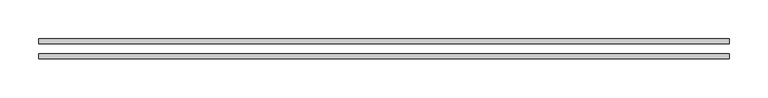
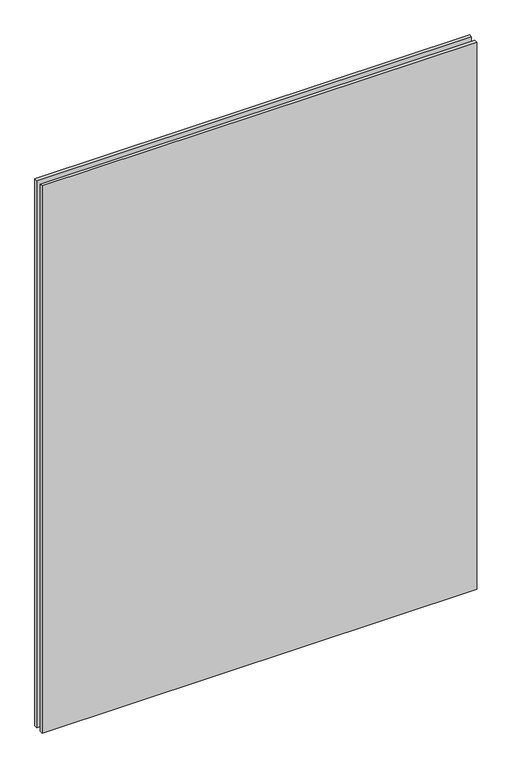
"""IFC4 building model written with IfcOpenShell, lengths in millimetres: proxy geometry, Window glass:Window glass:1:Window glass:1 : Window glass:Window glass:300352:337881:Window glass:1:Window glass:1 : Window glass:Window glass:300352:337881 : Window glass:Window glass:1:Window glass:1 : Window glass:Window glass:300352:337881:3 : Window glass:Window glass:1:Window glass:1 : Window glass:Window glass:300352:337881:Window glass:1:Window glass:1 : Window glass:Window glass:300352:337881 : Window glass:Window glass:1:Window glass:1 : Window glass:Window glass:300352:337881:301362."""

from ifc_helpers import new_model, si_unit, frame, origin, place, context, project, spatial, polyline, outline, extrude, source, transform, mapped, element, save


def generic_models_ca35c40b(model_context):
    return source(origin(), model_context, "Body", "SweptSolid", [
        extrude(outline(polyline([(593690.1661787, -579073.7163841), (592802.9478941, -579073.7163841), (592802.9478941, -579067.3663841), (593690.1661787, -579067.3663841), (593690.1661787, -579073.7163841)])), frame((0.0, 0.0, 2479.9705452), z_axis=(0.0, 0.0, 1.0), x_axis=(1.0, 0.0, 0.0)), (0.0, 0.0, 1.0), 1180.5089096),
        extrude(outline(polyline([(593690.1661787, -579054.6663841), (592802.9478941, -579054.6663841), (592802.9478941, -579048.3163841), (593690.1661787, -579048.3163841), (593690.1661787, -579054.6663841)])), frame((0.0, 0.0, 2479.9705452), z_axis=(0.0, 0.0, 1.0), x_axis=(1.0, 0.0, 0.0)), (0.0, 0.0, 1.0), 1180.5089096),
    ])


if __name__ == "__main__":
    model = new_model("IFC4")
    model_context = context("Model", 3, world=origin())
    ifc_project = project(units=[si_unit("LENGTHUNIT", "METRE", prefix="MILLI")], contexts=[model_context])
    site = spatial("IfcSite", under=ifc_project)
    building = spatial("IfcBuilding", under=site)
    placement = place(None, origin())
    generic_models_shape = generic_models_ca35c40b(model_context)
    element("IfcBuildingElementProxy", 1, Name="Window glass:Window glass:1:Window glass:1 : Window glass:Window glass:300352:337881:Window glass:1:Window glass:1 : Window glass:Window glass:300352:337881 : Window glass:Window glass:1:Window glass:1 : Window glass:Window glass:300352:337881:3 : Window glass:Window glass:1:Window glass:1 : Window glass:Window glass:300352:337881:Window glass:1:Window glass:1 : Window glass:Window glass:300352:337881 : Window glass:Window glass:1:Window glass:1 : Window glass:Window glass:300352:337881:301362", ObjectType="Window glass:Window glass:1:Window glass:1 : Window glass:Window glass:300352:337881:Window glass:1:Window glass:1 : Window glass:Window glass:300352:337881 : Window glass:Window glass:1:Window glass:1 : Window glass:Window glass:300352:337881:3 : Window glass:Window glass:1:Window glass:1 : Window glass:Window glass:300352:337881:Window glass:1:Window glass:1 : Window glass:Window glass:300352:337881 : Window glass:Window glass:1:Window glass:1 : Window glass:Window glass:300352:337881:301362", at=placement, inside=building, context=model_context, shape_type="MappedRepresentation", body=[
        mapped(generic_models_shape, transform((0.0, 0.0, 0.0), x_axis=(1.0, 0.0, 0.0), y_axis=(0.0, 1.0, 0.0), z_axis=(0.0, 0.0, 1.0))),
    ])
    save(model, "model.ifc")

# Revit data of these elements
# Type "Window glass:Window glass:1:Window glass:1 : Window glass:Window glass:300352:337881:Window glass:1:Window glass:1 : Window glass:Window glass:300352:337881 : Window glass:Window glass:1:Window glass:1 : Window glass:Window glass:300352:337881:3 : Window glass:Window glass:1:Window glass:1 : Window glass:Window glass:300352:337881:Window glass:1:Window glass:1 : Window glass:Window glass:300352:337881 : Window glass:Window glass:1:Window glass:1 : Window glass:Window glass:300352:337881:301362"
#   NameOverride = "Window glass:Window glass:1:Window glass:1 : Window glass:Window glass:300352:337881:Window glass:1:Window glass:1 : Window glass:Window glass:300352:337881 : Window glass:Window glass:1:Window glass:1 : Window glass:Window glass:300352:337881:301362"
#   ObjectTypeOverride = "Window glass:1:Window glass:1 : Window glass:Window glass:300352:337881 : Window glass:Window glass:1:Window glass:1 : Window glass:Window glass:300352:337881"
#   Reference = "Window glass"
#   Tag = "301362"
# Element 1 (IfcBuildingElementProxy, "Window glass:Window glass:1:Window glass:1 : Window glass:Window glass:300352:337881:Window glass:1:Window glass:1 : Window glass:Window glass:300352:337881 : Window glass:Window glass:1:Window glass:1 : Window glass:Window glass:300352:337881:3 : Window glass:Window glass:1:Window glass:1 : Window glass:Window glass:300352:337881:Window glass:1:Window glass:1 : Window glass:Window glass:300352:337881 : Window glass:Window glass:1:Window glass:1 : Window glass:Window glass:300352:337881:301362")
#   Materials on its faces: "INSULATED LOW-E GLAZING (SEE ELEVATIONS FOR U-FACTOR, SHGC, & LT)"
# Materials
#   "INSULATED LOW-E GLAZING (SEE ELEVATIONS FOR U-FACTOR, SHGC, & LT)": class "Unassigned", colour RGB 84 171 255, transparency 0, Cost = 0
